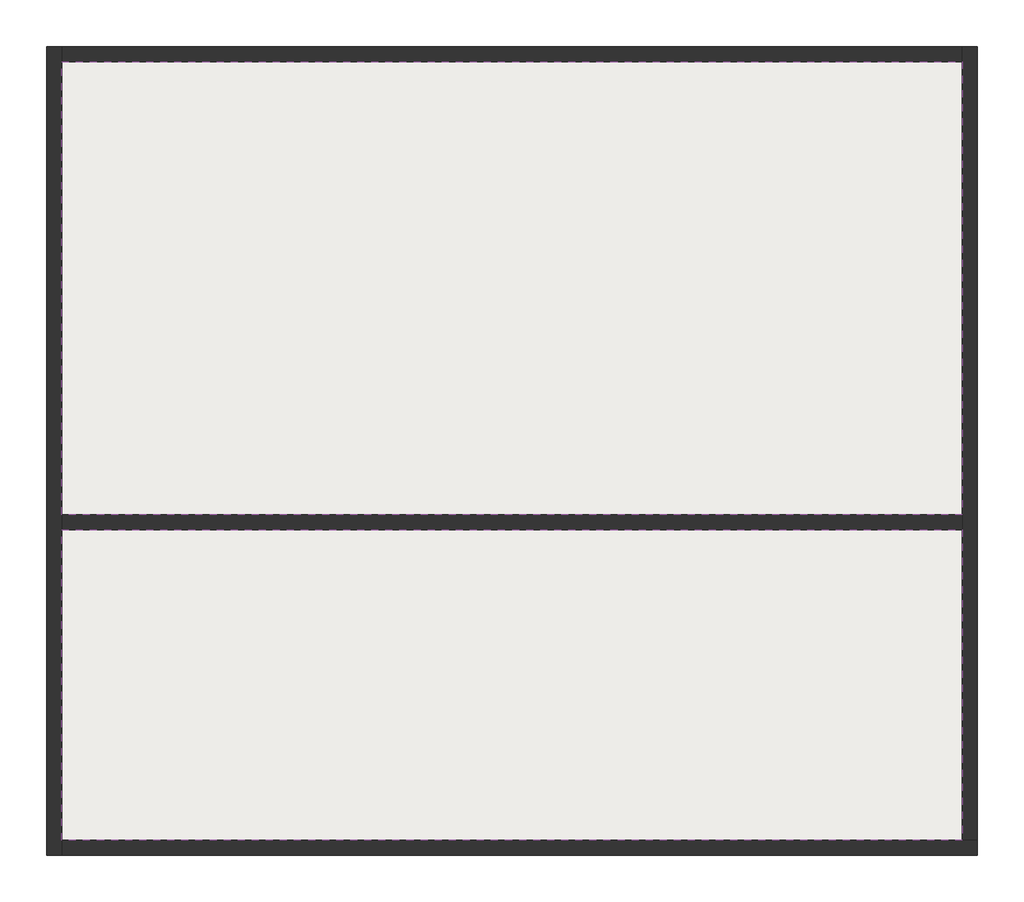
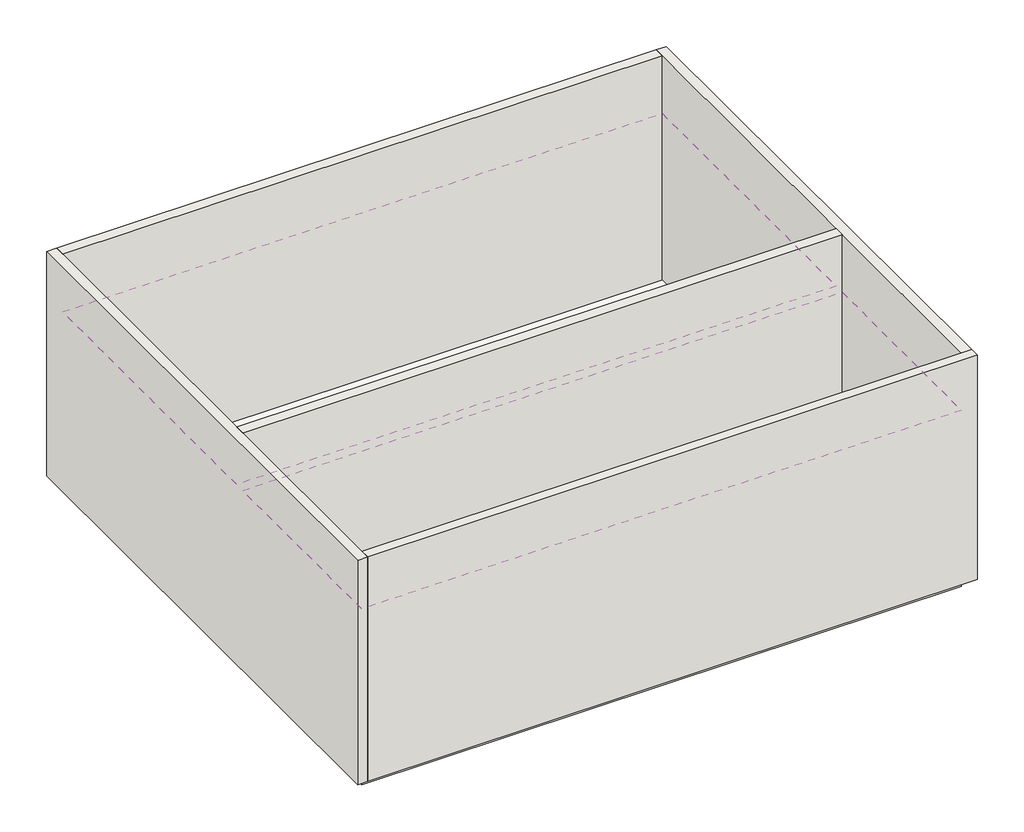
# One storey: 5 walls, 2 coverings, 1 slab.
"""IFC4 building model written with IfcOpenShell, lengths in millimetres."""

import ifcopenshell
import ifcopenshell.guid

model = None  # the IFC model being written
_history = None  # IfcOwnerHistory: only IFC2X3 demands one
_inside = {}  # id of a spatial element -> (the spatial element, [elements in it])
_under = {}  # id of a project, library or spatial element -> (it, [spatial elements below it])
_declared = {}  # id of a project -> (the project, [libraries it declares])
_typed = {}  # id of a type object -> (the type object, [elements of that type])
_made_of = {}  # id of a material, layer set ... -> (it, [elements and type objects made of it])


def new_model(schema):
    """Start an empty IFC model of exactly this schema.

    Asked for "IFC4X3", IfcOpenShell would pick the latest addendum, in which some entities
    have other attributes; the version numbers below select the first issue.
    IFC2X3 requires an IfcOwnerHistory on every rooted entity: one is made here for all.
    """
    global model, _history
    if schema == "IFC4X3":
        model = ifcopenshell.file(schema_version=(4, 3, 0, 0))
    else:
        model = ifcopenshell.file(schema=schema)
    _inside.clear()
    _under.clear()
    _declared.clear()
    _typed.clear()
    _made_of.clear()
    _history = None
    if model.schema == "IFC2X3":
        org = make("IfcOrganization", Name="unknown")
        user = make(
            "IfcPersonAndOrganization",
            ThePerson=make("IfcPerson", FamilyName="unknown"),
            TheOrganization=org,
        )
        app = make(
            "IfcApplication",
            ApplicationDeveloper=org,
            Version="unknown",
            ApplicationFullName="unknown",
            ApplicationIdentifier="unknown",
        )
        _history = make(
            "IfcOwnerHistory",
            OwningUser=user,
            OwningApplication=app,
            ChangeAction="ADDED",
            CreationDate=0,
        )
    return model


def make(cls, **values):
    """One entity of the class cls with the attributes given. An attribute that is None is left unset."""
    return model.create_entity(
        cls, **{name: value for name, value in values.items() if value is not None}
    )


def rooted(cls, **values):
    """An entity with a GlobalId (a new one), such as an element, a storey or a relation."""
    return make(cls, GlobalId=ifcopenshell.guid.new(), OwnerHistory=_history, **values)


def si_unit(unit_type, name, prefix=None):
    """IfcSIUnit, for example si_unit("LENGTHUNIT", "METRE", prefix="MILLI")."""
    return make("IfcSIUnit", UnitType=unit_type, Prefix=prefix, Name=name)


def assignment(units):
    """IfcUnitAssignment: the units of a project."""
    return None if units is None else make("IfcUnitAssignment", Units=units)


def point(xyz):
    """IfcCartesianPoint."""
    return None if xyz is None else make("IfcCartesianPoint", Coordinates=xyz)


def direction(xyz):
    """IfcDirection."""
    return None if xyz is None else make("IfcDirection", DirectionRatios=xyz)


def frame(location, z_axis=None, x_axis=None):
    """IfcAxis2Placement3D, a coordinate frame: its origin and axes. An axis left out is left unset."""
    return make(
        "IfcAxis2Placement3D",
        Location=point(location),
        Axis=direction(z_axis),
        RefDirection=direction(x_axis),
    )


def origin():
    """The frame at (0, 0, 0) with its axes left unset."""
    return frame((0.0, 0.0, 0.0))


def place(relative_to, where):
    """IfcLocalPlacement: puts the frame where relative to a parent placement (None: the world)."""
    return make(
        "IfcLocalPlacement", PlacementRelTo=relative_to, RelativePlacement=where
    )


def context(
    kind, dimensions, precision=None, world=None, true_north=None, identifier=None
):
    """IfcGeometricRepresentationContext, for example the 3D "Model" context."""
    return make(
        "IfcGeometricRepresentationContext",
        ContextIdentifier=identifier,
        ContextType=kind,
        CoordinateSpaceDimension=dimensions,
        Precision=precision,
        WorldCoordinateSystem=world,
        TrueNorth=true_north,
    )


def project(units=None, contexts=None):
    """IfcProject with its units and contexts."""
    return rooted(
        "IfcProject",
        Name="project",
        RepresentationContexts=contexts,
        UnitsInContext=assignment(units),
    )


def spatial(cls, under=None, at=None, **own):
    """A site, building, storey or space (cls), placed at a placement, below another one or the project."""
    s = rooted(cls, ObjectPlacement=at, **own)
    if under is not None:
        _under.setdefault(under.id(), (under, []))[1].append(s)
    return s


def polyline(points):
    """IfcPolyline through the points."""
    return make("IfcPolyline", Points=[point(p) for p in points])


def outline(outer, holes=None, kind="AREA"):
    """IfcArbitraryClosedProfileDef: a profile drawn as a closed curve; with holes, ...WithVoids."""
    if holes is None:
        return make("IfcArbitraryClosedProfileDef", ProfileType=kind, OuterCurve=outer)
    return make(
        "IfcArbitraryProfileDefWithVoids",
        ProfileType=kind,
        OuterCurve=outer,
        InnerCurves=holes,
    )


def extrude(swept, where, along, depth):
    """IfcExtrudedAreaSolid: the profile swept, set in the frame where, extruded along a direction by depth."""
    return make(
        "IfcExtrudedAreaSolid",
        SweptArea=swept,
        Position=where,
        ExtrudedDirection=direction(along),
        Depth=depth,
    )


def faces_of(points, faces, orient=None, outer=None):
    """IfcFace entities. A face is a list of loops; a loop is a list of indices into points, from 0.

    orient and outer hold one flag for each loop. By default every Orientation is true, the
    first loop of a face is its IfcFaceOuterBound and the others are IfcFaceBound.
    """
    made = []
    for i, loops in enumerate(faces):
        bounds = []
        for j, loop in enumerate(loops):
            is_outer = j == 0 if outer is None else outer[i][j]
            bounds.append(
                make(
                    "IfcFaceOuterBound" if is_outer else "IfcFaceBound",
                    Bound=make("IfcPolyLoop", Polygon=[points[k] for k in loop]),
                    Orientation=True if orient is None else orient[i][j],
                )
            )
        made.append(make("IfcFace", Bounds=bounds))
    return made


def faceted_brep(points, faces, orient=None, outer=None, voids=None):
    """IfcFacetedBrep: a solid bounded by flat faces; with voids (closed shells), ...WithVoids."""
    shared = [point(p) for p in points]
    hull = make("IfcClosedShell", CfsFaces=faces_of(shared, faces, orient, outer))
    if voids is None:
        return make("IfcFacetedBrep", Outer=hull)
    return make(
        "IfcFacetedBrepWithVoids",
        Outer=hull,
        Voids=[
            make(cls, CfsFaces=faces_of(shared, fs, o, b)) for cls, fs, o, b in voids
        ],
    )


def shape(context_of_items, identifier, shape_type, items):
    """IfcShapeRepresentation: the items that make up one representation, for example the "Body"."""
    return make(
        "IfcShapeRepresentation",
        ContextOfItems=context_of_items,
        RepresentationIdentifier=identifier,
        RepresentationType=shape_type,
        Items=items,
    )


def made_of(thing, what):
    """Note that an element or type object is made of a material, layer set ...; save() writes the relation."""
    if what is not None:
        _made_of.setdefault(what.id(), (what, []))[1].append(thing)
    return thing


def element(
    cls,
    number,
    at=None,
    inside=None,
    cuts=None,
    type_object=None,
    material=None,
    context=None,
    identifier="Body",
    shape_type=None,
    held_by="IfcProductDefinitionShape",
    body=None,
    shapes=None,
    **own,
):
    """One element of the class cls, such as IfcWall. Its Tag is "e" and its number.

    at: its placement. inside: the storey or other place that contains it. cuts: it is an
    opening in that element (IfcRelVoidsElement). A single representation is given by context,
    identifier, shape_type and body (its items); several are given by shapes. held_by: the class
    of the entity that holds the representations. save() writes the other relations.
    """
    e = rooted(cls, Tag="e%d" % number, ObjectPlacement=at, **own)
    if body is not None:
        shapes = [shape(context, identifier, shape_type, body)]
    if shapes is not None:
        e.Representation = make(held_by, Representations=shapes)
    if inside is not None:
        _inside.setdefault(inside.id(), (inside, []))[1].append(e)
    if cuts is not None:
        rooted(
            "IfcRelVoidsElement", RelatingBuildingElement=cuts, RelatedOpeningElement=e
        )
    if type_object is not None:
        _typed.setdefault(type_object.id(), (type_object, []))[1].append(e)
    return made_of(e, material)


def aggregate(whole, parts):
    """IfcRelAggregates: a whole, such as a stair, and the parts it consists of."""
    return rooted("IfcRelAggregates", RelatingObject=whole, RelatedObjects=parts)


def save(model, path):
    """Write the relations noted so far, then the file.

    IfcRelAggregates (storeys below a building ...), IfcRelContainedInSpatialStructure (elements
    in a storey), IfcRelDefinesByType, IfcRelAssociatesMaterial and IfcRelDeclares: one each for
    every whole, place, type object, material and project.
    """
    for whole, parts in _under.values():
        aggregate(whole, parts)
    for where, things in _inside.values():
        rooted(
            "IfcRelContainedInSpatialStructure",
            RelatedElements=things,
            RelatingStructure=where,
        )
    for kind, things in _typed.values():
        rooted("IfcRelDefinesByType", RelatedObjects=things, RelatingType=kind)
    for what, things in _made_of.values():
        rooted("IfcRelAssociatesMaterial", RelatedObjects=things, RelatingMaterial=what)
    for by, libraries in _declared.values():
        rooted("IfcRelDeclares", RelatingContext=by, RelatedDefinitions=libraries)
    model.write(path)


model = new_model("IFC4")

# Units and contexts
model_context = context("Model", 3, world=origin())
ifc_project = project(units=[si_unit("LENGTHUNIT", "METRE", prefix="MILLI")], contexts=[model_context])

# Site, building, storey
site = spatial("IfcSite", under=ifc_project)
building = spatial("IfcBuilding", under=site)
storey = spatial("IfcBuildingStorey", under=building, Name="レベル 2", Elevation=4000.0)

# Coverings
placement = place(None, origin())
element("IfcCovering", 1, ObjectType="グリッド 600x600mm", at=placement, inside=storey, context=model_context, shape_type="SweptSolid", body=[
    extrude(outline(polyline([(-1039.1497645, -1548.6940898), (-9889.1497645, -1548.6940898), (-9889.1497645, 2901.3059102), (-1039.1497645, 2901.3059102), (-1039.1497645, -1548.6940898)])), frame((0.0, 0.0, 6600.0), z_axis=(0.0, 0.0, 1.0), x_axis=(1.0, 0.0, 0.0)), (0.0, 0.0, 1.0), 52.0),
])
element("IfcCovering", 2, ObjectType="グリッド 600x600mm", at=placement, inside=storey, context=model_context, shape_type="SweptSolid", body=[
    extrude(outline(polyline([(-1039.1497645, -4748.6940898), (-9889.1497645, -4748.6940898), (-9889.1497645, -1698.6940898), (-1039.1497645, -1698.6940898), (-1039.1497645, -4748.6940898)])), frame((0.0, 0.0, 6600.0), z_axis=(0.0, 0.0, 1.0), x_axis=(1.0, 0.0, 0.0)), (0.0, 0.0, 1.0), 52.0),
])

# Slab
element("IfcSlab", 3, ObjectType="一般 150 mm", at=placement, inside=storey, context=model_context, shape_type="SweptSolid", body=[
    extrude(outline(polyline([(-1039.1497645, 2901.3059102), (-1039.1497645, -4748.6940898), (-9889.1497645, -4748.6940898), (-9889.1497645, 2901.3059102), (-1039.1497645, 2901.3059102)])), frame((0.0, 0.0, 3850.0), z_axis=(0.0, 0.0, 1.0), x_axis=(1.0, 0.0, 0.0)), (0.0, 0.0, 1.0), 150.0),
])

# Walls
element("IfcWall", 4, ObjectType="標準-150mm", at=placement, inside=storey, context=model_context, shape_type="Brep", body=[
    faceted_brep([(-10039.1497645, 3051.3059102, 4000.0), (-10039.1497645, -4898.6940898, 4000.0), (-10039.1497645, -4898.6940898, 7500.0), (-10039.1497645, 3051.3059102, 7500.0), (-9889.1497645, 3051.3059102, 4000.0), (-9889.1497645, 3051.3059102, 7500.0), (-9889.1497645, 2901.3059102, 7500.0), (-9889.1497645, -1548.6940898, 7500.0), (-9889.1497645, -1698.6940898, 7500.0), (-9889.1497645, -4748.6940898, 7500.0), (-9889.1497645, -4898.6940898, 7500.0), (-9889.1497645, -4898.6940898, 4000.0), (-9889.1497645, -4748.6940898, 4000.0), (-9889.1497645, -1698.6940898, 4000.0), (-9889.1497645, -1548.6940898, 4000.0), (-9889.1497645, 2901.3059102, 4000.0)], [[[0, 1, 2, 3]], [[4, 5, 6, 7, 8, 9, 10, 11, 12, 13, 14, 15]], [[1, 0, 4, 15, 14, 13, 12, 11]], [[3, 2, 10, 9, 8, 7, 6, 5]], [[0, 3, 5, 4]], [[2, 1, 11, 10]]]),
])
element("IfcWall", 5, ObjectType="標準-150mm", at=placement, inside=storey, context=model_context, shape_type="SweptSolid", body=[
    extrude(outline(polyline([(-1039.1497645, -1698.6940898), (-9889.1497645, -1698.6940898), (-9889.1497645, -1548.6940898), (-1039.1497645, -1548.6940898), (-1039.1497645, -1698.6940898)])), frame((0.0, 0.0, 4000.0), z_axis=(0.0, 0.0, 1.0), x_axis=(1.0, 0.0, 0.0)), (0.0, 0.0, 1.0), 3500.0),
])
element("IfcWall", 6, ObjectType="標準-150mm", at=placement, inside=storey, context=model_context, shape_type="Brep", body=[
    faceted_brep([(-889.1497645, -4748.6940898, 4000.0), (-889.1497645, 3051.3059102, 4000.0), (-889.1497645, 3051.3059102, 7500.0), (-889.1497645, -4748.6940898, 7500.0), (-1039.1497645, -4748.6940898, 4000.0), (-1039.1497645, -4748.6940898, 7500.0), (-1039.1497645, -1698.6940898, 7500.0), (-1039.1497645, -1548.6940898, 7500.0), (-1039.1497645, 2901.3059102, 7500.0), (-1039.1497645, 3051.3059102, 7500.0), (-1039.1497645, 3051.3059102, 4000.0), (-1039.1497645, 2901.3059102, 4000.0), (-1039.1497645, -1548.6940898, 4000.0), (-1039.1497645, -1698.6940898, 4000.0)], [[[0, 1, 2, 3]], [[4, 5, 6, 7, 8, 9, 10, 11, 12, 13]], [[1, 0, 4, 13, 12, 11, 10]], [[3, 2, 9, 8, 7, 6, 5]], [[2, 1, 10, 9]], [[0, 3, 5, 4]]]),
])
element("IfcWall", 7, ObjectType="標準-150mm", at=placement, inside=storey, context=model_context, shape_type="SweptSolid", body=[
    extrude(outline(polyline([(-9889.1497645, 3051.3059102), (-1039.1497645, 3051.3059102), (-1039.1497645, 2901.3059102), (-9889.1497645, 2901.3059102), (-9889.1497645, 3051.3059102)])), frame((0.0, 0.0, 4000.0), z_axis=(0.0, 0.0, 1.0), x_axis=(1.0, 0.0, 0.0)), (0.0, 0.0, 1.0), 3500.0),
])
element("IfcWall", 8, ObjectType="標準-150mm", at=placement, inside=storey, context=model_context, shape_type="Brep", body=[
    faceted_brep([(-9889.1497645, -4898.6940898, 4000.0), (-889.1497645, -4898.6940898, 4000.0), (-889.1497645, -4898.6940898, 7500.0), (-9889.1497645, -4898.6940898, 7500.0), (-9889.1497645, -4748.6940898, 4000.0), (-9889.1497645, -4748.6940898, 7500.0), (-1039.1497645, -4748.6940898, 7500.0), (-889.1497645, -4748.6940898, 7500.0), (-889.1497645, -4748.6940898, 4000.0), (-1039.1497645, -4748.6940898, 4000.0)], [[[0, 1, 2, 3]], [[4, 5, 6, 7, 8, 9]], [[1, 0, 4, 9, 8]], [[3, 2, 7, 6, 5]], [[0, 3, 5, 4]], [[2, 1, 8, 7]]]),
])

save(model, "model.ifc")

# Revit data of these elements
# Type "グリッド 600x600mm"
#   built-in parameter 1002203 = 1 (stored number, unit not read)
#   built-in parameter 1002202 = 1 (stored number, unit not read)
#   Layers, outside or top first: 36 mm no material (function 1); 16 mm "天井タイル 600 x 600" (function 5)
# Type "一般 150 mm"
#   Function = 0
#   Layers, outside or top first: 150 mm no material (function 1)
# Type "標準-150mm"
#   Layers, outside or top first: 150 mm no material (function 1)
# Elements 1, 2 (IfcCovering, "グリッド 600x600mm")
#   Height Offset From Level = 2600 mm
#   Phase Created = 新しい建設
#   Materials on its faces: "天井タイル 600 x 600"
# Element 3 (IfcSlab, "一般 150 mm")
#   Height Offset From Level = 0 mm
#   Phase Created = 新しい建設
# Elements 4, 5, 6, 7, 8 (IfcWall, "標準-150mm")
#   Top Offset = 3500 mm
#   Base Offset = 0 mm
#   wall height = 3500 mm
#   Phase Created = 新しい建設
#   Base Constraint = レベル 2
#   Top Constraint = レベル 2
#   Materials on its faces: "既定の壁"
# Materials
#   "天井タイル 600 x 600": class "一般", colour RGB 235 235 235, transparency 0, Description = "吸音天井タイル", Cost = 0
#   "既定の壁": class "その他", colour RGB 127 127 127, transparency 0, Cost = 0
